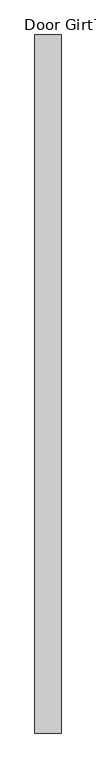
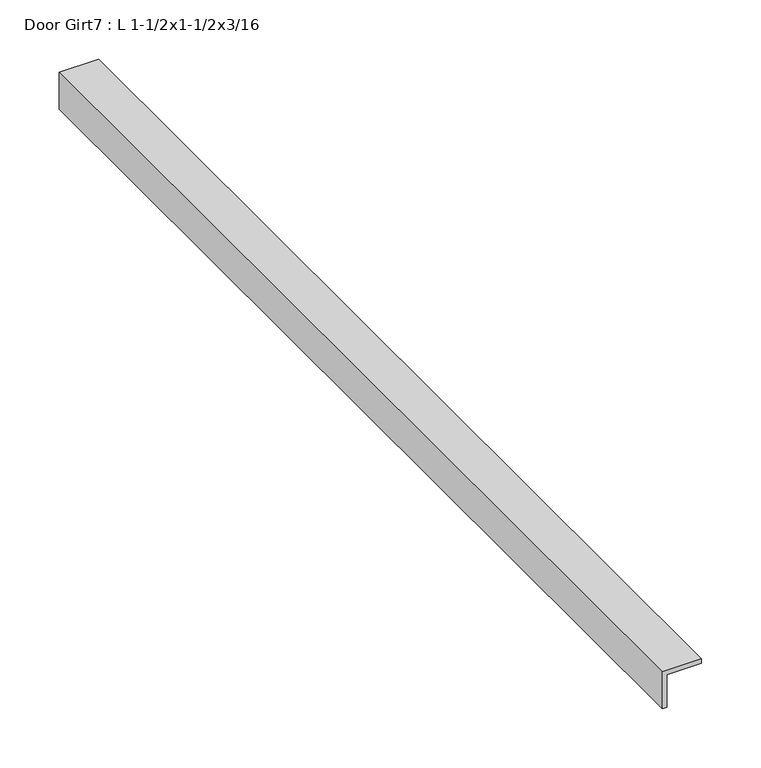
"""IFC4 building model written with IfcOpenShell, lengths in millimetres: proxy geometry, Door Girt7 : L 1-1/2x1-1/2x3/16."""

from ifc_helpers import new_model, si_unit, frame, origin, place, context, project, spatial, polyline, outline, extrude, source, transform, mapped, element, save


def door_girt7_l_1_1_2x1_1_2x3_16_18399394(model_context):
    return source(origin(), model_context, "Body", "SweptSolid", [
        extrude(outline(polyline([(812.8, 587403.9934739), (812.8, 587365.8934739), (774.7, 587365.8934739), (774.7, 587370.6559739), (808.0375, 587370.6559739), (808.0375, 587403.9934739), (812.8, 587403.9934739)])), frame((0.0, -533937.9163841, 0.0), z_axis=(0.0, 1.0, 0.0), x_axis=(0.0, 0.0, 1.0)), (0.0, 0.0, 1.0), 1016.0),
    ])


if __name__ == "__main__":
    model = new_model("IFC4")
    model_context = context("Model", 3, world=origin())
    ifc_project = project(units=[si_unit("LENGTHUNIT", "METRE", prefix="MILLI")], contexts=[model_context])
    site = spatial("IfcSite", under=ifc_project)
    building = spatial("IfcBuilding", under=site)
    placement = place(None, origin())
    door_girt7_l_1_1_2x1_1_2x3_16_shape = door_girt7_l_1_1_2x1_1_2x3_16_18399394(model_context)
    element("IfcBuildingElementProxy", 1, Name="Door Girt7 : L 1-1/2x1-1/2x3/16", ObjectType="Door Girt7 : L 1-1/2x1-1/2x3/16", at=placement, inside=building, context=model_context, shape_type="MappedRepresentation", body=[
        mapped(door_girt7_l_1_1_2x1_1_2x3_16_shape, transform((0.0, 0.0, 0.0), x_axis=(1.0, 0.0, 0.0), y_axis=(0.0, 1.0, 0.0), z_axis=(0.0, 0.0, 1.0))),
    ])
    save(model, "model.ifc")

# Revit data of these elements
# Element 1 (IfcBuildingElementProxy, "Door Girt7 : L 1-1/2x1-1/2x3/16")
#   Materials on its faces: "1-1/2\"X1-1/2\" GALV. STL L"
# Materials
#   "1-1/2\"X1-1/2\" GALV. STL L": class "Generic", colour RGB 211 211 207, transparency 0, Cost = 0
